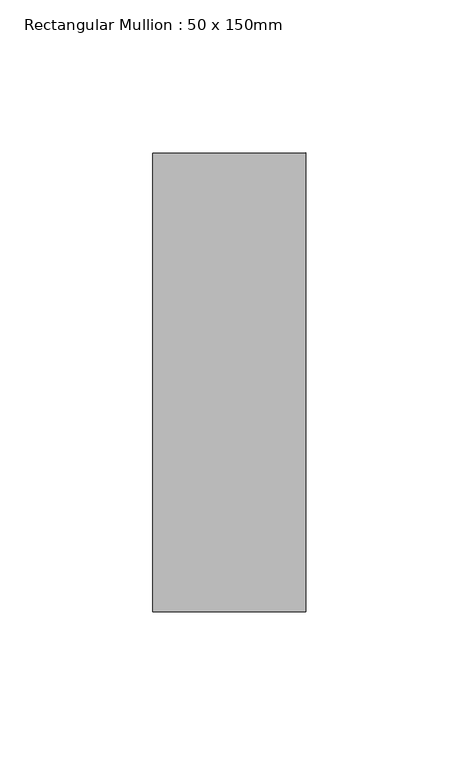
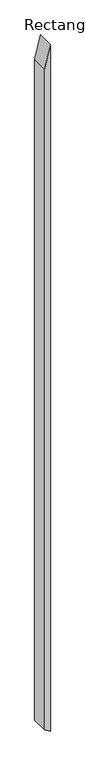
"""IFC4 building model written with IfcOpenShell, lengths in millimetres: member geometry, Rectangular Mullion : 50 x 150mm."""

import ifcopenshell
import ifcopenshell.guid

model = None  # the IFC model being written
_history = None  # IfcOwnerHistory: only IFC2X3 demands one
_inside = {}  # id of a spatial element -> (the spatial element, [elements in it])
_under = {}  # id of a project, library or spatial element -> (it, [spatial elements below it])
_declared = {}  # id of a project -> (the project, [libraries it declares])
_typed = {}  # id of a type object -> (the type object, [elements of that type])
_made_of = {}  # id of a material, layer set ... -> (it, [elements and type objects made of it])


def new_model(schema):
    """Start an empty IFC model of exactly this schema.

    Asked for "IFC4X3", IfcOpenShell would pick the latest addendum, in which some entities
    have other attributes; the version numbers below select the first issue.
    IFC2X3 requires an IfcOwnerHistory on every rooted entity: one is made here for all.
    """
    global model, _history
    if schema == "IFC4X3":
        model = ifcopenshell.file(schema_version=(4, 3, 0, 0))
    else:
        model = ifcopenshell.file(schema=schema)
    _inside.clear()
    _under.clear()
    _declared.clear()
    _typed.clear()
    _made_of.clear()
    _history = None
    if model.schema == "IFC2X3":
        org = make("IfcOrganization", Name="unknown")
        user = make(
            "IfcPersonAndOrganization",
            ThePerson=make("IfcPerson", FamilyName="unknown"),
            TheOrganization=org,
        )
        app = make(
            "IfcApplication",
            ApplicationDeveloper=org,
            Version="unknown",
            ApplicationFullName="unknown",
            ApplicationIdentifier="unknown",
        )
        _history = make(
            "IfcOwnerHistory",
            OwningUser=user,
            OwningApplication=app,
            ChangeAction="ADDED",
            CreationDate=0,
        )
    return model


def make(cls, **values):
    """One entity of the class cls with the attributes given. An attribute that is None is left unset."""
    return model.create_entity(
        cls, **{name: value for name, value in values.items() if value is not None}
    )


def rooted(cls, **values):
    """An entity with a GlobalId (a new one), such as an element, a storey or a relation."""
    return make(cls, GlobalId=ifcopenshell.guid.new(), OwnerHistory=_history, **values)


def si_unit(unit_type, name, prefix=None):
    """IfcSIUnit, for example si_unit("LENGTHUNIT", "METRE", prefix="MILLI")."""
    return make("IfcSIUnit", UnitType=unit_type, Prefix=prefix, Name=name)


def assignment(units):
    """IfcUnitAssignment: the units of a project."""
    return None if units is None else make("IfcUnitAssignment", Units=units)


def point(xyz):
    """IfcCartesianPoint."""
    return None if xyz is None else make("IfcCartesianPoint", Coordinates=xyz)


def direction(xyz):
    """IfcDirection."""
    return None if xyz is None else make("IfcDirection", DirectionRatios=xyz)


def frame(location, z_axis=None, x_axis=None):
    """IfcAxis2Placement3D, a coordinate frame: its origin and axes. An axis left out is left unset."""
    return make(
        "IfcAxis2Placement3D",
        Location=point(location),
        Axis=direction(z_axis),
        RefDirection=direction(x_axis),
    )


def origin():
    """The frame at (0, 0, 0) with its axes left unset."""
    return frame((0.0, 0.0, 0.0))


def place(relative_to, where):
    """IfcLocalPlacement: puts the frame where relative to a parent placement (None: the world)."""
    return make(
        "IfcLocalPlacement", PlacementRelTo=relative_to, RelativePlacement=where
    )


def context(
    kind, dimensions, precision=None, world=None, true_north=None, identifier=None
):
    """IfcGeometricRepresentationContext, for example the 3D "Model" context."""
    return make(
        "IfcGeometricRepresentationContext",
        ContextIdentifier=identifier,
        ContextType=kind,
        CoordinateSpaceDimension=dimensions,
        Precision=precision,
        WorldCoordinateSystem=world,
        TrueNorth=true_north,
    )


def project(units=None, contexts=None):
    """IfcProject with its units and contexts."""
    return rooted(
        "IfcProject",
        Name="project",
        RepresentationContexts=contexts,
        UnitsInContext=assignment(units),
    )


def spatial(cls, under=None, at=None, **own):
    """A site, building, storey or space (cls), placed at a placement, below another one or the project."""
    s = rooted(cls, ObjectPlacement=at, **own)
    if under is not None:
        _under.setdefault(under.id(), (under, []))[1].append(s)
    return s


def polyline(points):
    """IfcPolyline through the points."""
    return make("IfcPolyline", Points=[point(p) for p in points])


def outline(outer, holes=None, kind="AREA"):
    """IfcArbitraryClosedProfileDef: a profile drawn as a closed curve; with holes, ...WithVoids."""
    if holes is None:
        return make("IfcArbitraryClosedProfileDef", ProfileType=kind, OuterCurve=outer)
    return make(
        "IfcArbitraryProfileDefWithVoids",
        ProfileType=kind,
        OuterCurve=outer,
        InnerCurves=holes,
    )


def extrude(swept, where, along, depth):
    """IfcExtrudedAreaSolid: the profile swept, set in the frame where, extruded along a direction by depth."""
    return make(
        "IfcExtrudedAreaSolid",
        SweptArea=swept,
        Position=where,
        ExtrudedDirection=direction(along),
        Depth=depth,
    )


def shape(context_of_items, identifier, shape_type, items):
    """IfcShapeRepresentation: the items that make up one representation, for example the "Body"."""
    return make(
        "IfcShapeRepresentation",
        ContextOfItems=context_of_items,
        RepresentationIdentifier=identifier,
        RepresentationType=shape_type,
        Items=items,
    )


def source(mapping_origin, context_of_items, identifier, shape_type, items):
    """IfcRepresentationMap: a shape defined once, which mapped items show again and again."""
    return make(
        "IfcRepresentationMap",
        MappingOrigin=mapping_origin,
        MappedRepresentation=shape(context_of_items, identifier, shape_type, items),
    )


def transform(
    local_origin,
    x_axis=None,
    y_axis=None,
    z_axis=None,
    scale=None,
    scale2=None,
    scale3=None,
    uniform=True,
):
    """IfcCartesianTransformationOperator3D, or its non-uniform kind. x_axis, y_axis, z_axis: its Axis1, 2, 3."""
    if uniform:
        return make(
            "IfcCartesianTransformationOperator3D",
            Axis1=direction(x_axis),
            Axis2=direction(y_axis),
            LocalOrigin=point(local_origin),
            Scale=scale,
            Axis3=direction(z_axis),
        )
    return make(
        "IfcCartesianTransformationOperator3DnonUniform",
        Axis1=direction(x_axis),
        Axis2=direction(y_axis),
        LocalOrigin=point(local_origin),
        Scale=scale,
        Axis3=direction(z_axis),
        Scale2=scale2,
        Scale3=scale3,
    )


def mapped(mapping_source, mapping_target):
    """IfcMappedItem: shows the shape of a source again, moved by a transform."""
    return make(
        "IfcMappedItem", MappingSource=mapping_source, MappingTarget=mapping_target
    )


def made_of(thing, what):
    """Note that an element or type object is made of a material, layer set ...; save() writes the relation."""
    if what is not None:
        _made_of.setdefault(what.id(), (what, []))[1].append(thing)
    return thing


def element(
    cls,
    number,
    at=None,
    inside=None,
    cuts=None,
    type_object=None,
    material=None,
    context=None,
    identifier="Body",
    shape_type=None,
    held_by="IfcProductDefinitionShape",
    body=None,
    shapes=None,
    **own,
):
    """One element of the class cls, such as IfcWall. Its Tag is "e" and its number.

    at: its placement. inside: the storey or other place that contains it. cuts: it is an
    opening in that element (IfcRelVoidsElement). A single representation is given by context,
    identifier, shape_type and body (its items); several are given by shapes. held_by: the class
    of the entity that holds the representations. save() writes the other relations.
    """
    e = rooted(cls, Tag="e%d" % number, ObjectPlacement=at, **own)
    if body is not None:
        shapes = [shape(context, identifier, shape_type, body)]
    if shapes is not None:
        e.Representation = make(held_by, Representations=shapes)
    if inside is not None:
        _inside.setdefault(inside.id(), (inside, []))[1].append(e)
    if cuts is not None:
        rooted(
            "IfcRelVoidsElement", RelatingBuildingElement=cuts, RelatedOpeningElement=e
        )
    if type_object is not None:
        _typed.setdefault(type_object.id(), (type_object, []))[1].append(e)
    return made_of(e, material)


def aggregate(whole, parts):
    """IfcRelAggregates: a whole, such as a stair, and the parts it consists of."""
    return rooted("IfcRelAggregates", RelatingObject=whole, RelatedObjects=parts)


def save(model, path):
    """Write the relations noted so far, then the file.

    IfcRelAggregates (storeys below a building ...), IfcRelContainedInSpatialStructure (elements
    in a storey), IfcRelDefinesByType, IfcRelAssociatesMaterial and IfcRelDeclares: one each for
    every whole, place, type object, material and project.
    """
    for whole, parts in _under.values():
        aggregate(whole, parts)
    for where, things in _inside.values():
        rooted(
            "IfcRelContainedInSpatialStructure",
            RelatedElements=things,
            RelatingStructure=where,
        )
    for kind, things in _typed.values():
        rooted("IfcRelDefinesByType", RelatedObjects=things, RelatingType=kind)
    for what, things in _made_of.values():
        rooted("IfcRelAssociatesMaterial", RelatedObjects=things, RelatingMaterial=what)
    for by, libraries in _declared.values():
        rooted("IfcRelDeclares", RelatingContext=by, RelatedDefinitions=libraries)
    model.write(path)


def rectangular_mullion_50_x_150mm_3e1f935b(model_context):
    return source(origin(), model_context, "Body", "SweptSolid", [
        extrude(outline(polyline([(0.0, 0.0), (-213.3099575, -50.0), (-6299.3378645, -50.0), (-6328.6389336, 0.0), (0.0, 0.0)])), frame((0.0, -75.0, 0.0), z_axis=(0.0, 1.0, 0.0), x_axis=(0.0, 0.0, 1.0)), (0.0, 0.0, 1.0), 150.0),
    ])


if __name__ == "__main__":
    model = new_model("IFC4")
    model_context = context("Model", 3, world=origin())
    ifc_project = project(units=[si_unit("LENGTHUNIT", "METRE", prefix="MILLI")], contexts=[model_context])
    site = spatial("IfcSite", under=ifc_project)
    building = spatial("IfcBuilding", under=site)
    placement = place(None, origin())
    rectangular_mullion_50_x_150mm_shape = rectangular_mullion_50_x_150mm_3e1f935b(model_context)
    element("IfcMember", 1, ObjectType="Rectangular Mullion : 50 x 150mm", at=placement, inside=building, context=model_context, shape_type="MappedRepresentation", body=[
        mapped(rectangular_mullion_50_x_150mm_shape, transform((0.0, 0.0, 0.0), x_axis=(1.0, 0.0, 0.0), y_axis=(0.0, 1.0, 0.0), z_axis=(0.0, 0.0, 1.0))),
    ])
    save(model, "model.ifc")

# Revit data of these elements
# Type "Rectangular Mullion : 50 x 150mm"
#   built-in parameter 1007304 = 0.492126 (stored number, unit not read)
#   built-in parameter 1007301 = 0.082021 (stored number, unit not read)
#   built-in parameter 1007300 = 0.082021 (stored number, unit not read)
# Element 1 (IfcMember, "Rectangular Mullion : 50 x 150mm")
#   Materials on its faces: "Metal - Aluminium"
# Materials
#   "Metal - Aluminium": class "Metal", colour RGB 247 247 247, transparency 0
